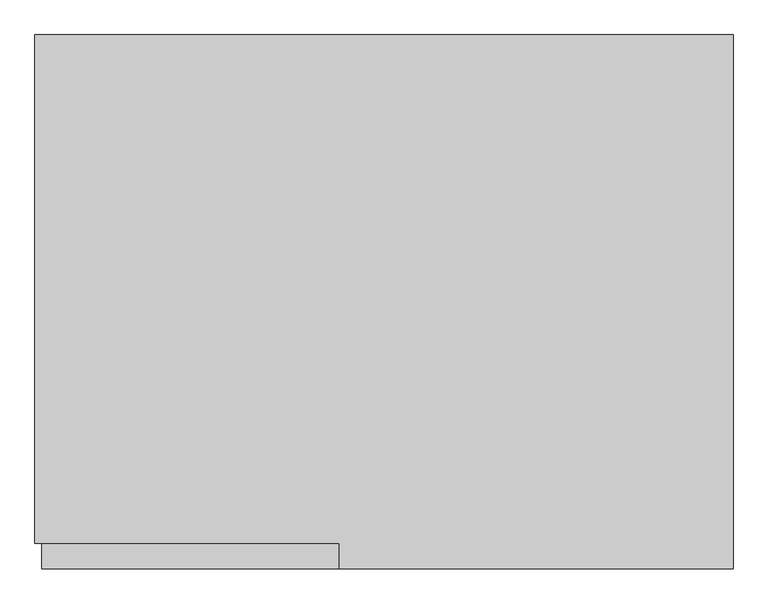
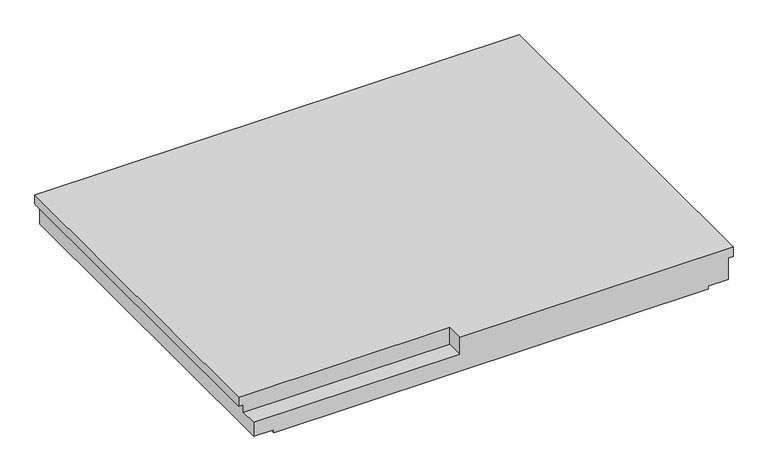
"""IFC4 building model written with IfcOpenShell, lengths in millimetres: stair geometry, NLRS_24_GM_UN_rechthoekig bordes prefab zonder oplegnok-AV_gen_rsf : prefab bordes_gen__2300x3005."""

from ifc_helpers import new_model, si_unit, origin, place, context, project, spatial, faceted_brep, source, transform, mapped, element, save


def stair_1f0cb1f1(model_context):
    return source(origin(), model_context, "Body", "Brep", [
        faceted_brep([(1502.5, -2300.0, 0.0), (1502.5, -2300.0, -60.0), (1502.5, 0.0, -60.0), (1502.5, 0.0, 0.0), (-192.5, -2300.0, 0.0), (-192.5, -2190.0, 0.0), (-192.5, -2190.0, -110.0), (-192.5, -2300.0, -110.0), (-1502.5, 0.0, 0.0), (-1502.5, 0.0, -60.0), (-1502.5, -2190.0, -60.0), (-1502.5, -2190.0, 0.0), (-1472.5, -2300.0, -110.0), (-1472.5, -2300.0, -200.0), (-1347.5, -2300.0, -200.0), (-1347.5, -2300.0, -220.0), (1347.5, -2300.0, -220.0), (1347.5, -2300.0, -200.0), (1472.5, -2300.0, -200.0), (1472.5, -2300.0, -60.0), (-1472.5, -2190.0, -110.0), (-1472.5, -2190.0, -60.0), (1472.5, 0.0, -60.0), (1472.5, 0.0, -200.0), (1347.5, 0.0, -200.0), (1347.5, 0.0, -220.0), (-1347.5, 0.0, -220.0), (-1347.5, 0.0, -200.0), (-1472.5, 0.0, -200.0), (-1472.5, 0.0, -60.0)], [[[0, 1, 2, 3]], [[4, 5, 6, 7]], [[8, 9, 10, 11]], [[12, 13, 14, 15, 16, 17, 18, 19, 1, 0, 4, 7]], [[7, 6, 20, 12]], [[11, 10, 21, 20, 6, 5]], [[11, 5, 4, 0, 3, 8]], [[8, 3, 2, 22, 23, 24, 25, 26, 27, 28, 29, 9]], [[26, 25, 16, 15]], [[21, 10, 9, 29]], [[13, 12, 20, 21, 29, 28]], [[28, 27, 14, 13]], [[27, 26, 15, 14]], [[22, 2, 1, 19]], [[19, 18, 23, 22]], [[18, 17, 24, 23]], [[17, 16, 25, 24]]]),
    ])


if __name__ == "__main__":
    model = new_model("IFC4")
    model_context = context("Model", 3, world=origin())
    ifc_project = project(units=[si_unit("LENGTHUNIT", "METRE", prefix="MILLI")], contexts=[model_context])
    site = spatial("IfcSite", under=ifc_project)
    building = spatial("IfcBuilding", under=site)
    placement = place(None, origin())
    stair_shape = stair_1f0cb1f1(model_context)
    element("IfcStair", 1, ObjectType="NLRS_24_GM_UN_rechthoekig bordes prefab zonder oplegnok-AV_gen_rsf : prefab bordes_gen__2300x3005", at=placement, inside=building, context=model_context, shape_type="MappedRepresentation", body=[
        mapped(stair_shape, transform((0.0, 0.0, 0.0), x_axis=(1.0, 0.0, 0.0), y_axis=(0.0, 1.0, 0.0), z_axis=(0.0, 0.0, 1.0))),
    ])
    save(model, "model.ifc")

# Revit data of these elements
# Type "NLRS_24_GM_UN_rechthoekig bordes prefab zonder oplegnok-AV_gen_rsf : prefab bordes_gen__2300x3005"
#   IfcExportAs = "IfcStair"
#   Type Comments = " "
#   Model = " "
#   Manufacturer = " "
#   Description = "rechthoekig bordes prefab\r\n1930x4395"
#   Assembly Code = "24.15"
#   Width = 3005 mm
#   Thickness = 220 mm
#   Perimeter = 10610 mm
#   NLRS_C_lengte_02 = 1310 mm
#   NLRS_C_lengte_01 = 1310 mm
#   NLRS_C_hoogte_02 = 110 mm
#   NLRS_C_hoogte_01 = 110 mm
#   NLRS_C_diepte_04 = 2300 mm
#   NLRS_C_diepte_03 = 2300 mm
#   NLRS_C_diepte_02 = 110 mm
#   NLRS_C_diepte_01 = 110 mm
#   Length = 2300 mm
#   Default Elevation = 1219.2 mm
#   Area = 6.9115 m²
#   NLRS_C_materiaal = NLRS_f2_beton prefab_gen_rsf
#   Keynote = ""
# Element 1 (IfcStair, "NLRS_24_GM_UN_rechthoekig bordes prefab zonder oplegnok-AV_gen_rsf : prefab bordes_gen__2300x3005")
#   Materials on its faces: "NLRS_f2_beton prefab_gen_rsf"
# Materials
#   "NLRS_f2_beton prefab_gen_rsf": class "F - Niet gebakken kunststeen", colour RGB 129 133 118, transparency 0, Keynote = "f2", Manufacturer = "Revit Standards Foundation", URL = "www.revitstandards.org", Description = "beton prefab", Cost = 0
